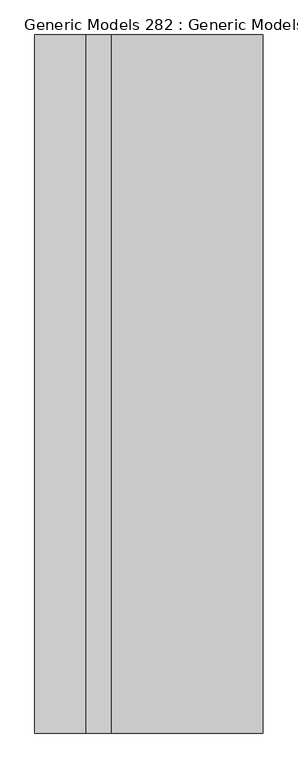
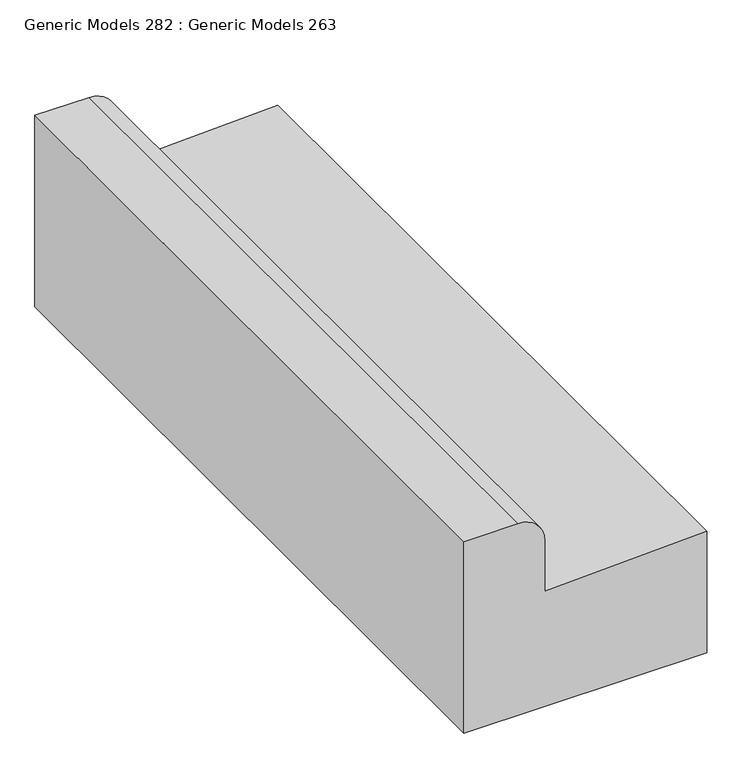
"""IFC4 building model written with IfcOpenShell, lengths in millimetres: proxy geometry, Generic Models 282 : Generic Models 263."""

from ifc_helpers import new_model, si_unit, point, frame, frame_2d, origin, place, context, project, spatial, polyline, circle_curve, trimmed, segment, composite_curve, outline, extrude, source, transform, mapped, element, save


def generic_models_282_generic_models_263_cc0d5e36(model_context):
    return source(origin(), model_context, "Body", "SweptSolid", [
        extrude(outline(composite_curve([segment(polyline([(0.0, 91681.5797726), (0.0, 91579.9797726), (-381.0, 91579.9797726), (-381.0, 92037.1797726), (-139.7, 92037.1797726), (-152.4, 91732.3797726), (-50.8, 91732.3797726)]), True, "CONTINUOUS"), segment(trimmed(circle_curve(frame_2d((-50.8, 91681.5797726)), 50.8), [point((-50.8, 91732.3797726))], [point((0.0, 91681.5797726))], False, "CARTESIAN"), True, "CONTINUOUS")], self_intersect=False)), frame((0.0, 2106.5727422, 0.0), z_axis=(0.0, 1.0, 0.0), x_axis=(0.0, 0.0, 1.0)), (0.0, 0.0, 1.0), 1397.4322547),
    ])


if __name__ == "__main__":
    model = new_model("IFC4")
    model_context = context("Model", 3, world=origin())
    ifc_project = project(units=[si_unit("LENGTHUNIT", "METRE", prefix="MILLI")], contexts=[model_context])
    site = spatial("IfcSite", under=ifc_project)
    building = spatial("IfcBuilding", under=site)
    placement = place(None, origin())
    generic_models_282_generic_models_263_shape = generic_models_282_generic_models_263_cc0d5e36(model_context)
    element("IfcBuildingElementProxy", 1, Name="Generic Models 282 : Generic Models 263", ObjectType="Generic Models 282 : Generic Models 263", at=placement, inside=building, context=model_context, shape_type="MappedRepresentation", body=[
        mapped(generic_models_282_generic_models_263_shape, transform((0.0, 0.0, 0.0), x_axis=(1.0, 0.0, 0.0), y_axis=(0.0, 1.0, 0.0), z_axis=(0.0, 0.0, 1.0))),
    ])
    save(model, "model.ifc")

# Revit data of these elements
# Element 1 (IfcBuildingElementProxy, "Generic Models 282 : Generic Models 263")
#   Materials on its faces: "CONCRETE CURB"
# Materials
#   "CONCRETE CURB": class "Concrete", colour RGB 191 191 191, transparency 0, Description = "Cast-in-place concrete", Cost = 0
